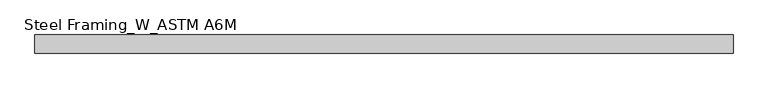
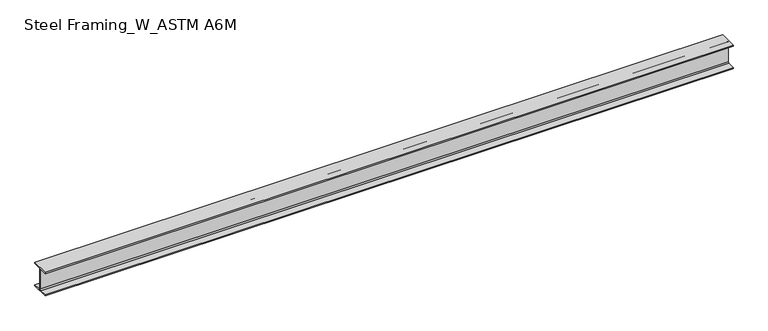
"""IFC4 building model written with IfcOpenShell, lengths in millimetres: beam geometry, Steel Framing_W_ASTM A6M : H_SB_AR_S02_W360x91_B3."""

from ifc_helpers import new_model, si_unit, point, frame, frame_2d, origin, place, context, project, spatial, polyline, circle_curve, trimmed, segment, composite_curve, outline, extrude, source, transform, mapped, element, save


def steel_framing_w_astm_a6m_37bec3ec(model_context):
    return source(origin(), model_context, "Body", "SweptSolid", [
        extrude(outline(composite_curve([segment(polyline([(127.0, -160.1), (127.0, -176.5), (-127.0, -176.5), (-127.0, -160.1), (-19.865, -160.1)]), True, "CONTINUOUS"), segment(trimmed(circle_curve(frame_2d((-19.865, -145.0)), 15.1), [point((-19.865, -160.1))], [point((-4.765, -145.0))], True, "CARTESIAN"), True, "CONTINUOUS"), segment(polyline([(-4.765, -145.0), (-4.765, 145.0)]), True, "CONTINUOUS"), segment(trimmed(circle_curve(frame_2d((-19.865, 145.0)), 15.1), [point((-4.765, 145.0))], [point((-19.865, 160.1))], True, "CARTESIAN"), True, "CONTINUOUS"), segment(polyline([(-19.865, 160.1), (-127.0, 160.1), (-127.0, 176.5), (127.0, 176.5), (127.0, 160.1), (19.865, 160.1)]), True, "CONTINUOUS"), segment(trimmed(circle_curve(frame_2d((19.865, 145.0)), 15.1), [point((19.865, 160.1))], [point((4.765, 145.0))], True, "CARTESIAN"), True, "CONTINUOUS"), segment(polyline([(4.765, 145.0), (4.765, -145.0)]), True, "CONTINUOUS"), segment(trimmed(circle_curve(frame_2d((19.865, -145.0)), 15.1), [point((4.765, -145.0))], [point((19.865, -160.1))], True, "CARTESIAN"), True, "CONTINUOUS"), segment(polyline([(19.865, -160.1), (127.0, -160.1)]), True, "CONTINUOUS")], self_intersect=False)), frame((-4885.8, 0.0, 0.0), z_axis=(1.0, 0.0, 0.0), x_axis=(0.0, 1.0, 0.0)), (0.0, 0.0, 1.0), 9771.6),
    ])


if __name__ == "__main__":
    model = new_model("IFC4")
    model_context = context("Model", 3, world=origin())
    ifc_project = project(units=[si_unit("LENGTHUNIT", "METRE", prefix="MILLI")], contexts=[model_context])
    site = spatial("IfcSite", under=ifc_project)
    building = spatial("IfcBuilding", under=site)
    placement = place(None, origin())
    steel_framing_w_astm_a6m_shape = steel_framing_w_astm_a6m_37bec3ec(model_context)
    element("IfcBeam", 1, ObjectType="Steel Framing_W_ASTM A6M : H_SB_AR_S02_W360x91_B3", at=placement, inside=building, context=model_context, shape_type="MappedRepresentation", body=[
        mapped(steel_framing_w_astm_a6m_shape, transform((0.0, 0.0, 0.0), x_axis=(1.0, 0.0, 0.0), y_axis=(0.0, 1.0, 0.0), z_axis=(0.0, 0.0, 1.0))),
    ])
    save(model, "model.ifc")

# Revit data of these elements
# Type "Steel Framing_W_ASTM A6M : H_SB_AR_S02_W360x91_B3"
#   Type Mark = "B3"
#   Section Name Key = "W14x61"
#   Width = 25.4 cm
#   Web Thickness = 0.953 cm
#   Web Fillet = 1.51 cm
#   Warping Constant = 1260000.0 cm⁶
#   Torsional Moment of Inertia = 91.20 cm⁴
#   Section Area = 115.0 cm²
#   Plastic Modulus weak axis = 537.0 cm³
#   Plastic Modulus strong axis = 1670.0 cm³
#   Perimeter = 1.68 m²/m
#   Nominal Weight = 91.00 kgf/m
#   Moment of Inertia weak axis = 4450.00 cm⁴
#   Moment of Inertia strong axis = 26600.00 cm⁴
#   Height = 35.3 cm
#   Flange Thickness = 1.64 cm
#   Elastic Modulus weak axis = 352.0 cm³
#   Elastic Modulus strong axis = 1510.0 cm³
#   Centroid Vertical = 17.65 cm
#   Centroid Horizontal = 12.7 cm
#   Length [instance default] = 1500 mm
#   Structural Material [instance default] = Steel, 45-345
#   Bolt Spacing = 0
#   Assembly Code = ""
# Element 1 (IfcBeam, "Steel Framing_W_ASTM A6M : H_SB_AR_S02_W360x91_B3")
#   Materials on its faces: "Steel, 45-345"
# Materials
#   "Steel, 45-345": class "Metal", colour RGB 189 187 185, transparency 0, Description = "Steel 345 MPa", Cost = 0
